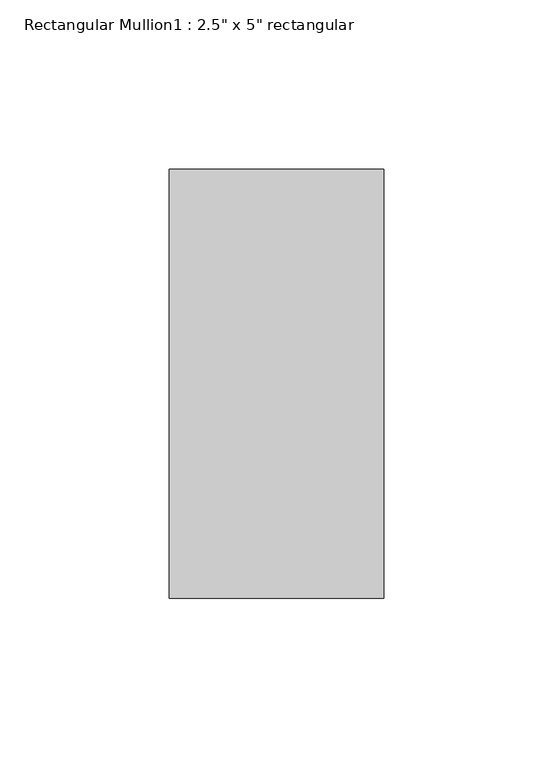
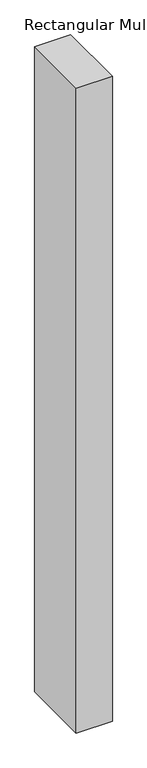
"""IFC4 building model written with IfcOpenShell, lengths in millimetres: member geometry."""

import ifcopenshell
import ifcopenshell.guid

model = None  # the IFC model being written
_history = None  # IfcOwnerHistory: only IFC2X3 demands one
_inside = {}  # id of a spatial element -> (the spatial element, [elements in it])
_under = {}  # id of a project, library or spatial element -> (it, [spatial elements below it])
_declared = {}  # id of a project -> (the project, [libraries it declares])
_typed = {}  # id of a type object -> (the type object, [elements of that type])
_made_of = {}  # id of a material, layer set ... -> (it, [elements and type objects made of it])


def new_model(schema):
    """Start an empty IFC model of exactly this schema.

    Asked for "IFC4X3", IfcOpenShell would pick the latest addendum, in which some entities
    have other attributes; the version numbers below select the first issue.
    IFC2X3 requires an IfcOwnerHistory on every rooted entity: one is made here for all.
    """
    global model, _history
    if schema == "IFC4X3":
        model = ifcopenshell.file(schema_version=(4, 3, 0, 0))
    else:
        model = ifcopenshell.file(schema=schema)
    _inside.clear()
    _under.clear()
    _declared.clear()
    _typed.clear()
    _made_of.clear()
    _history = None
    if model.schema == "IFC2X3":
        org = make("IfcOrganization", Name="unknown")
        user = make(
            "IfcPersonAndOrganization",
            ThePerson=make("IfcPerson", FamilyName="unknown"),
            TheOrganization=org,
        )
        app = make(
            "IfcApplication",
            ApplicationDeveloper=org,
            Version="unknown",
            ApplicationFullName="unknown",
            ApplicationIdentifier="unknown",
        )
        _history = make(
            "IfcOwnerHistory",
            OwningUser=user,
            OwningApplication=app,
            ChangeAction="ADDED",
            CreationDate=0,
        )
    return model


def make(cls, **values):
    """One entity of the class cls with the attributes given. An attribute that is None is left unset."""
    return model.create_entity(
        cls, **{name: value for name, value in values.items() if value is not None}
    )


def rooted(cls, **values):
    """An entity with a GlobalId (a new one), such as an element, a storey or a relation."""
    return make(cls, GlobalId=ifcopenshell.guid.new(), OwnerHistory=_history, **values)


def si_unit(unit_type, name, prefix=None):
    """IfcSIUnit, for example si_unit("LENGTHUNIT", "METRE", prefix="MILLI")."""
    return make("IfcSIUnit", UnitType=unit_type, Prefix=prefix, Name=name)


def assignment(units):
    """IfcUnitAssignment: the units of a project."""
    return None if units is None else make("IfcUnitAssignment", Units=units)


def point(xyz):
    """IfcCartesianPoint."""
    return None if xyz is None else make("IfcCartesianPoint", Coordinates=xyz)


def direction(xyz):
    """IfcDirection."""
    return None if xyz is None else make("IfcDirection", DirectionRatios=xyz)


def frame(location, z_axis=None, x_axis=None):
    """IfcAxis2Placement3D, a coordinate frame: its origin and axes. An axis left out is left unset."""
    return make(
        "IfcAxis2Placement3D",
        Location=point(location),
        Axis=direction(z_axis),
        RefDirection=direction(x_axis),
    )


def origin():
    """The frame at (0, 0, 0) with its axes left unset."""
    return frame((0.0, 0.0, 0.0))


def place(relative_to, where):
    """IfcLocalPlacement: puts the frame where relative to a parent placement (None: the world)."""
    return make(
        "IfcLocalPlacement", PlacementRelTo=relative_to, RelativePlacement=where
    )


def context(
    kind, dimensions, precision=None, world=None, true_north=None, identifier=None
):
    """IfcGeometricRepresentationContext, for example the 3D "Model" context."""
    return make(
        "IfcGeometricRepresentationContext",
        ContextIdentifier=identifier,
        ContextType=kind,
        CoordinateSpaceDimension=dimensions,
        Precision=precision,
        WorldCoordinateSystem=world,
        TrueNorth=true_north,
    )


def project(units=None, contexts=None):
    """IfcProject with its units and contexts."""
    return rooted(
        "IfcProject",
        Name="project",
        RepresentationContexts=contexts,
        UnitsInContext=assignment(units),
    )


def spatial(cls, under=None, at=None, **own):
    """A site, building, storey or space (cls), placed at a placement, below another one or the project."""
    s = rooted(cls, ObjectPlacement=at, **own)
    if under is not None:
        _under.setdefault(under.id(), (under, []))[1].append(s)
    return s


def polyline(points):
    """IfcPolyline through the points."""
    return make("IfcPolyline", Points=[point(p) for p in points])


def outline(outer, holes=None, kind="AREA"):
    """IfcArbitraryClosedProfileDef: a profile drawn as a closed curve; with holes, ...WithVoids."""
    if holes is None:
        return make("IfcArbitraryClosedProfileDef", ProfileType=kind, OuterCurve=outer)
    return make(
        "IfcArbitraryProfileDefWithVoids",
        ProfileType=kind,
        OuterCurve=outer,
        InnerCurves=holes,
    )


def extrude(swept, where, along, depth):
    """IfcExtrudedAreaSolid: the profile swept, set in the frame where, extruded along a direction by depth."""
    return make(
        "IfcExtrudedAreaSolid",
        SweptArea=swept,
        Position=where,
        ExtrudedDirection=direction(along),
        Depth=depth,
    )


def shape(context_of_items, identifier, shape_type, items):
    """IfcShapeRepresentation: the items that make up one representation, for example the "Body"."""
    return make(
        "IfcShapeRepresentation",
        ContextOfItems=context_of_items,
        RepresentationIdentifier=identifier,
        RepresentationType=shape_type,
        Items=items,
    )


def source(mapping_origin, context_of_items, identifier, shape_type, items):
    """IfcRepresentationMap: a shape defined once, which mapped items show again and again."""
    return make(
        "IfcRepresentationMap",
        MappingOrigin=mapping_origin,
        MappedRepresentation=shape(context_of_items, identifier, shape_type, items),
    )


def transform(
    local_origin,
    x_axis=None,
    y_axis=None,
    z_axis=None,
    scale=None,
    scale2=None,
    scale3=None,
    uniform=True,
):
    """IfcCartesianTransformationOperator3D, or its non-uniform kind. x_axis, y_axis, z_axis: its Axis1, 2, 3."""
    if uniform:
        return make(
            "IfcCartesianTransformationOperator3D",
            Axis1=direction(x_axis),
            Axis2=direction(y_axis),
            LocalOrigin=point(local_origin),
            Scale=scale,
            Axis3=direction(z_axis),
        )
    return make(
        "IfcCartesianTransformationOperator3DnonUniform",
        Axis1=direction(x_axis),
        Axis2=direction(y_axis),
        LocalOrigin=point(local_origin),
        Scale=scale,
        Axis3=direction(z_axis),
        Scale2=scale2,
        Scale3=scale3,
    )


def mapped(mapping_source, mapping_target):
    """IfcMappedItem: shows the shape of a source again, moved by a transform."""
    return make(
        "IfcMappedItem", MappingSource=mapping_source, MappingTarget=mapping_target
    )


def made_of(thing, what):
    """Note that an element or type object is made of a material, layer set ...; save() writes the relation."""
    if what is not None:
        _made_of.setdefault(what.id(), (what, []))[1].append(thing)
    return thing


def element(
    cls,
    number,
    at=None,
    inside=None,
    cuts=None,
    type_object=None,
    material=None,
    context=None,
    identifier="Body",
    shape_type=None,
    held_by="IfcProductDefinitionShape",
    body=None,
    shapes=None,
    **own,
):
    """One element of the class cls, such as IfcWall. Its Tag is "e" and its number.

    at: its placement. inside: the storey or other place that contains it. cuts: it is an
    opening in that element (IfcRelVoidsElement). A single representation is given by context,
    identifier, shape_type and body (its items); several are given by shapes. held_by: the class
    of the entity that holds the representations. save() writes the other relations.
    """
    e = rooted(cls, Tag="e%d" % number, ObjectPlacement=at, **own)
    if body is not None:
        shapes = [shape(context, identifier, shape_type, body)]
    if shapes is not None:
        e.Representation = make(held_by, Representations=shapes)
    if inside is not None:
        _inside.setdefault(inside.id(), (inside, []))[1].append(e)
    if cuts is not None:
        rooted(
            "IfcRelVoidsElement", RelatingBuildingElement=cuts, RelatedOpeningElement=e
        )
    if type_object is not None:
        _typed.setdefault(type_object.id(), (type_object, []))[1].append(e)
    return made_of(e, material)


def aggregate(whole, parts):
    """IfcRelAggregates: a whole, such as a stair, and the parts it consists of."""
    return rooted("IfcRelAggregates", RelatingObject=whole, RelatedObjects=parts)


def save(model, path):
    """Write the relations noted so far, then the file.

    IfcRelAggregates (storeys below a building ...), IfcRelContainedInSpatialStructure (elements
    in a storey), IfcRelDefinesByType, IfcRelAssociatesMaterial and IfcRelDeclares: one each for
    every whole, place, type object, material and project.
    """
    for whole, parts in _under.values():
        aggregate(whole, parts)
    for where, things in _inside.values():
        rooted(
            "IfcRelContainedInSpatialStructure",
            RelatedElements=things,
            RelatingStructure=where,
        )
    for kind, things in _typed.values():
        rooted("IfcRelDefinesByType", RelatedObjects=things, RelatingType=kind)
    for what, things in _made_of.values():
        rooted("IfcRelAssociatesMaterial", RelatedObjects=things, RelatingMaterial=what)
    for by, libraries in _declared.values():
        rooted("IfcRelDeclares", RelatingContext=by, RelatedDefinitions=libraries)
    model.write(path)


def member_7ac431fd(model_context):
    return source(origin(), model_context, "Body", "SweptSolid", [
        extrude(outline(polyline([(0.0, 63.5), (0.0, -63.5), (-63.5, -63.5), (-63.5, 63.5), (0.0, 63.5)])), frame((0.0, 0.0, -1202.1401937), z_axis=(0.0, 0.0, 1.0), x_axis=(1.0, 0.0, 0.0)), (0.0, 0.0, 1.0), 1202.1401937),
    ])


if __name__ == "__main__":
    model = new_model("IFC4")
    model_context = context("Model", 3, world=origin())
    ifc_project = project(units=[si_unit("LENGTHUNIT", "METRE", prefix="MILLI")], contexts=[model_context])
    site = spatial("IfcSite", under=ifc_project)
    building = spatial("IfcBuilding", under=site)
    placement = place(None, origin())
    member_shape = member_7ac431fd(model_context)
    element("IfcMember", 1, ObjectType="Rectangular Mullion1 : 2.5\" x 5\" rectangular", at=placement, inside=building, context=model_context, shape_type="MappedRepresentation", body=[
        mapped(member_shape, transform((0.0, 0.0, 0.0), x_axis=(1.0, 0.0, 0.0), y_axis=(0.0, 1.0, 0.0), z_axis=(0.0, 0.0, 1.0))),
    ])
    save(model, "model.ifc")

# Revit data of these elements
# Type "Rectangular Mullion1 : 2.5\" x 5\" rectangular"
#   built-in parameter 1007304 = 0.416667 (stored number, unit not read)
#   built-in parameter 1007301 = 0.104167 (stored number, unit not read)
#   built-in parameter 1007300 = 0.104167 (stored number, unit not read)
# Element 1 (IfcMember, "Rectangular Mullion1 : 2.5\" x 5\" rectangular")
#   Materials on its faces: "support-frame"
# Materials
#   "support-frame": class "Unassigned", colour RGB 233 233 233, transparency 0, Cost = 0
